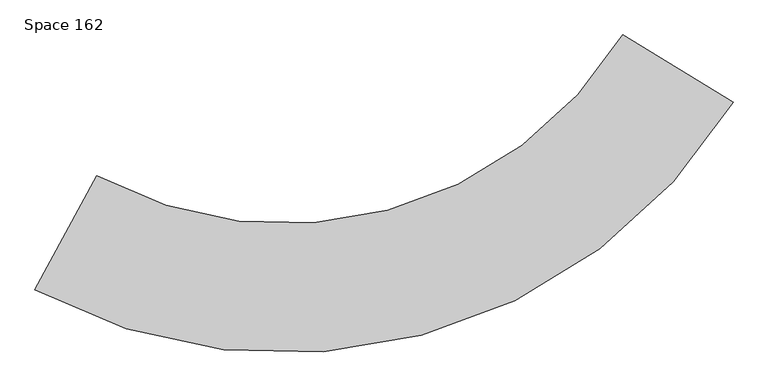
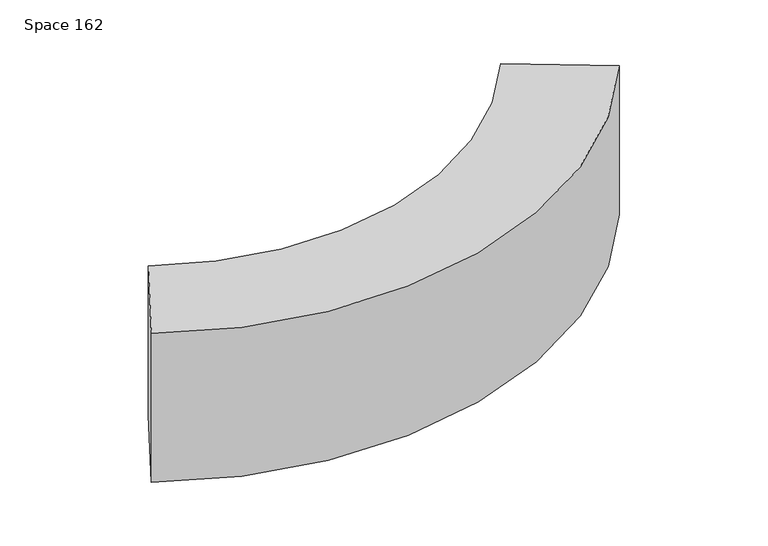
"""IFC4 building model written with IfcOpenShell, lengths in millimetres: proxy geometry, Space 162."""

from ifc_helpers import new_model, si_unit, point, frame, frame_2d, origin, place, context, project, spatial, polyline, circle_curve, trimmed, segment, composite_curve, outline, extrude, source, transform, mapped, element, save


def space_162_5186a034(model_context):
    return source(origin(), model_context, "Body", "SweptSolid", [
        extrude(outline(composite_curve([segment(polyline([(-19468.9209178, -29336.1215561), (-17779.6702242, -30371.2957125)]), True, "CONTINUOUS"), segment(trimmed(circle_curve(frame_2d((-24639.5440345, -26167.559635)), 8045.45), [point((-17779.6702242, -30371.2957125))], [point((-28478.5009822, -33238.0387741))], False, "CARTESIAN"), True, "CONTINUOUS"), segment(polyline([(-28478.5009822, -33238.0387741), (-27533.1540464, -31496.9263105)]), True, "CONTINUOUS"), segment(trimmed(circle_curve(frame_2d((-24639.5440345, -26167.559635)), 6064.25), [point((-27533.1540464, -31496.9263105))], [point((-19468.9209178, -29336.1215561))], True, "CARTESIAN"), True, "CONTINUOUS")], self_intersect=False)), frame((0.0, 0.0, 3810.0), z_axis=(0.0, 0.0, 1.0), x_axis=(1.0, 0.0, 0.0)), (0.0, 0.0, 1.0), 3048.0),
    ])


if __name__ == "__main__":
    model = new_model("IFC4")
    model_context = context("Model", 3, world=origin())
    ifc_project = project(units=[si_unit("LENGTHUNIT", "METRE", prefix="MILLI")], contexts=[model_context])
    site = spatial("IfcSite", under=ifc_project)
    building = spatial("IfcBuilding", under=site)
    placement = place(None, origin())
    space_162_shape = space_162_5186a034(model_context)
    element("IfcBuildingElementProxy", 1, Name="Space 162", ObjectType="Space 162", at=placement, inside=building, context=model_context, shape_type="MappedRepresentation", body=[
        mapped(space_162_shape, transform((0.0, 0.0, 0.0), x_axis=(1.0, 0.0, 0.0), y_axis=(0.0, 1.0, 0.0), z_axis=(0.0, 0.0, 1.0))),
    ])
    save(model, "model.ifc")

# Revit data of these elements
# Element 1 (IfcBuildingElementProxy, "Space 162")
#   Materials on its faces: "Render Material 255-255-255"
# Materials
#   "Render Material 255-255-255": class "Unassigned", colour RGB 255 255 255, transparency 0
